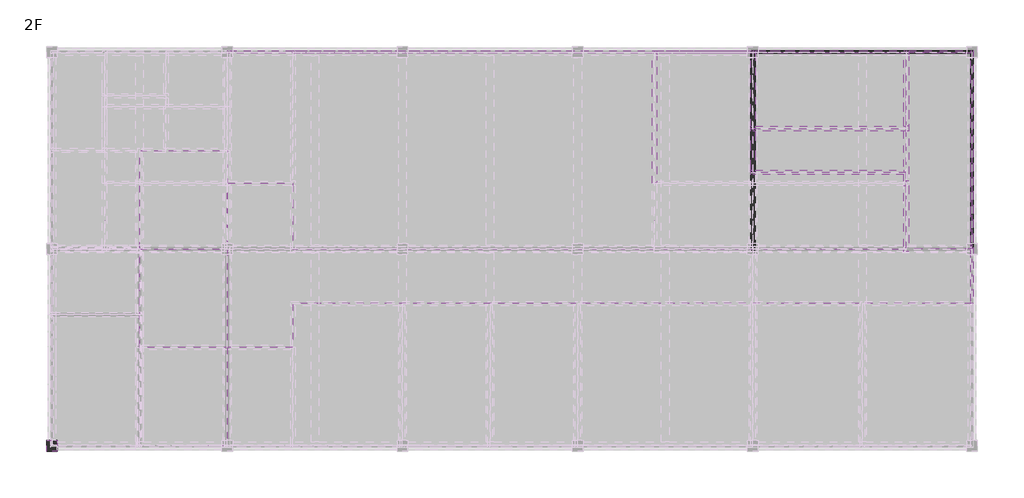
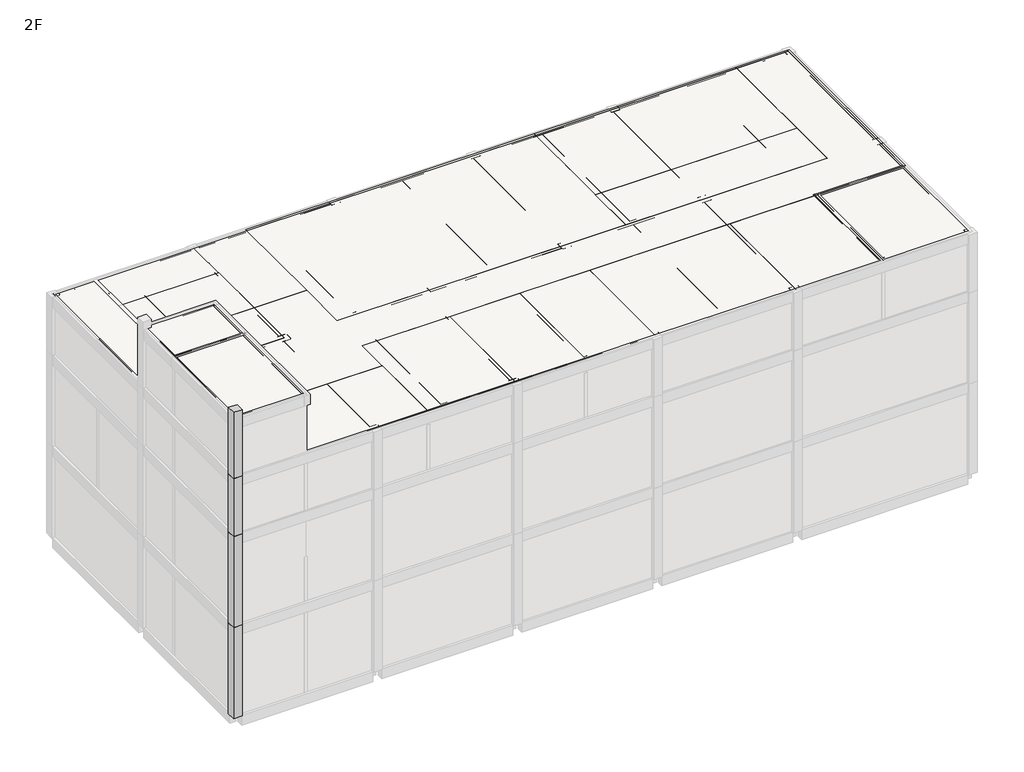
# One storey, part 3 of 7: 58 slabs, 19 walls, 4 columns.
# Revit data of these elements (continued)
# Element 71 (IfcWall, "WA211_Exterior-Cement Brick-90mm") (continued)
#   Base Offset = 0 mm
#   Unconnected Height = 3500 mm
#   wall height = 3500 mm
#   Phase Created = New Construction
#   Base Constraint = 4F
#   Materials on its faces: "Default Wall", "A04AS164-00001_Plastering_Ext", "A04AS164-00002_Plastering_Int"
# Element 73 (IfcWall, "WA221_Interior-Cement Block-190mm")
#   Top Offset = 0 mm
#   Base Offset = 0 mm
#   Unconnected Height = 5500 mm
#   wall height = 5500 mm
#   Phase Created = New Construction
#   Base Constraint = 2F
#   Materials on its faces: "A04AS164-00002_Plastering_Int", "Default Wall", "A04AS164-00001_Plastering_Ext"
# Element 74 (IfcWall, "WA221_Interior-Cement Block-190mm")
#   Top Offset = 0 mm
#   Base Offset = 0 mm
#   Unconnected Height = 3400 mm
#   wall height = 3400 mm
#   Phase Created = New Construction
#   Base Constraint = 3F
#   Materials on its faces: "Default Wall", "A04AS164-00002_Plastering_Int", "A04AS164-00001_Plastering_Ext"
# Element 75 (IfcWall, "WA221_Interior-Cement Block-190mm")
#   Top Offset = 0 mm
#   Base Offset = 0 mm
#   Unconnected Height = 3400 mm
#   wall height = 3400 mm
#   Phase Created = New Construction
#   Base Constraint = 3F
#   Materials on its faces: "Default Wall", "A04AS164-00002_Plastering_Int"
# Elements 76, 78 (IfcWall, "WA221_Interior-Cement Block-190mm")
#   Top Offset = 0 mm
#   Base Offset = 0 mm
#   Unconnected Height = 2700 mm
#   wall height = 2700 mm
#   Phase Created = New Construction
#   Base Constraint = 3F
#   Materials on its faces: "A04AS164-00002_Plastering_Int", "Default Wall"
# Element 77 (IfcWall, "WA221_Interior-Cement Block-190mm")
#   Top Offset = 0 mm
#   Base Offset = 0 mm
#   Unconnected Height = 2700 mm
#   wall height = 2700 mm
#   Phase Created = New Construction
#   Base Constraint = 3F
#   Materials on its faces: "Default Wall", "A04AS164-00002_Plastering_Int", "A04AS164-00001_Plastering_Ext"
# Elements 79, 80 (IfcWall, "WA221_Interior-Cement Block-190mm")
#   Top Offset = 0 mm
#   Base Offset = 0 mm
#   Unconnected Height = 2700 mm
#   wall height = 2700 mm
#   Phase Created = New Construction
#   Base Constraint = 4F
#   Materials on its faces: "Default Wall", "A04AS164-00002_Plastering_Int", "A04AS164-00001_Plastering_Ext"
# Element 81 (IfcWall, "WA221_Interior-Cement Block-190mm")
#   Top Offset = 0 mm
#   Base Offset = 0 mm
#   Unconnected Height = 2700 mm
#   wall height = 2700 mm
#   Phase Created = New Construction
#   Base Constraint = 4F
#   Materials on its faces: "A04AS164-00002_Plastering_Int", "Default Wall"
# Materials
#   "A03AE056-00001_Bitumen/Bituminous/Asphalt Coating": class "Generic", colour RGB 17 17 17, transparency 0, Description = "Damp-proofing", W00) Work Master Code = "A03AE056-00001", W01) Work Master_Lv1 = "Concrete Work", W02) Work Master_Lv2 = "Concrete Protective Coating (U/G)", W03) Work Master_Spec.1 = "Bitumen/Bituminous/Asphalt Coating", Cost = 0
#   "A03AC035-00001_Form Work (3 times in use)_Flat": class "Wood", colour RGB 149 120 74, transparency 0, Description = "Plywood", W00) Work Master Code = "A03AC035-00001", W01) Work Master_Lv1 = "Concrete Work", W02) Work Master_Lv2 = "Substructure Work", W03) Work Master_Spec.1 = "Form Work (3 times in use)", W04) Work Master_Spec.2 = "Flat Form", W05) Work Master_Spec.3 = "Dressed Lumber, Plywood or Steel Form(Wood Planks are not Allowed) incl. Chamfer", Cost = 0
#   "A03AC032-00007_Structural Concrete_Type1_25MPa-30Mpa": class "Concrete", colour RGB 176 176 176, transparency 0, Keynote = "09910.A1", Description = "Reinf. Conc.", W00) Work Master Code = "A03AC032-00007", W01) Work Master_Lv1 = "Concrete Work", W02) Work Master_Lv2 = "Substructure Work", W03) Work Master_Spec.1 = "Structural Concrete", W04) Work Master_Spec.2 = "Cement Type-1", W05) Work Master_Spec.3 = "25MPa < F'c (Cylinder Strength) ≤ 30MPa", Cost = 0
#   "14200-030101_Concrete Pouring": class "Concrete", colour RGB 176 176 176, transparency 0, Description = "Reinf. Conc.", W00) Work Master Code = "14200-030101", W01) Work Master_Lv1 = "Concrete Work", W02) Work Master_Lv2 = "Building/Shelter Foundation Work", W03) Work Master_Spec.1 = "Concrete Pouring", W04) Work Master_Spec.2 = "F'c (Cylinder Strength) > 35MPa", W05) Work Master_Spec.3 = "Cement Type-1", Cost = 0
#   "A04AL081-00001_Skirt_Acrylic Emulsion Paint": class "Finish", colour RGB 128 128 64, transparency 0, Description = "Plastic", W00) Work Master Code = "A04AL081-00001", W01) Work Master_Lv1 = "Finishing Work", W02) Work Master_Lv2 = "Painting Work", W03) Work Master_Spec.1 = "Skirt Painting", W04) Work Master_Spec.2 = "Acrylic Emulsion Paint", W05) Work Master_Spec.3 = "100mm≤H<150mm", Cost = 0
#   "A04AL077-00001_Ext Wall Painting_Acrylic Emulsion Paint": class "Finish", colour RGB 128 128 64, transparency 0, Description = "Plastic", W00) Work Master Code = "A04AL077-00001", W01) Work Master_Lv1 = "Finishing Work", W02) Work Master_Lv2 = "Painting Work", W03) Work Master_Spec.1 = "External Wall Painting", W04) Work Master_Spec.2 = "Acrylic Emulsion Paint", Cost = 0
#   "A04AS164-00001_Plastering_Ext": class "Concrete", colour RGB 183 186 184, transparency 0, W00) Work Master Code = "A04AS164-00001", W01) Work Master_Lv1 = "Finishing Work", W02) Work Master_Lv2 = "Plastering Work", W03) Work Master_Spec.1 = "Plastering", W04) Work Master_Spec.2 = "for External Masonry Wall", Cost = 0
#   "A04AK073-00001_Concrete Brick_0.5B": class "Concrete", colour RGB 180 180 180, transparency 0, Description = "Conc. Block", W00) Work Master Code = "A04AK073-00001", W01) Work Master_Lv1 = "Finishing Work", W02) Work Master_Lv2 = "Masonry Work", W03) Work Master_Spec.1 = "Concrete Brick", W04) Work Master_Spec.2 = "[0.5B] w/ All Reinf.(Lath, Steel Tie, Anchor Bar, Mortar, ETC.), Filler, Sealant, Lintel/Sill for Opening, ETC.", Cost = 0
#   "A04AS164-00002_Plastering_Int": class "Concrete", colour RGB 183 186 184, transparency 0, Description = "LATEX PAINT ON THK.15 CEMENT PLASTER", W00) Work Master Code = "A04AS164-00002", W01) Work Master_Lv1 = "Finishing Work", W02) Work Master_Lv2 = "Plastering Work", W03) Work Master_Spec.1 = "Plastering", W04) Work Master_Spec.2 = "for Internal Masonry Wall", Cost = 0
#   "A04AL078-00002_Int Wall Painting_Water Emulsion Paint": class "Finish", colour RGB 128 128 64, transparency 0, Description = "Plastic", W00) Work Master Code = "A04AL078-00002", W01) Work Master_Lv1 = "Finishing Work", W02) Work Master_Lv2 = "Painting Work", W03) Work Master_Spec.1 = "Internal Wall Painting", W04) Work Master_Spec.2 = "Water Emulsion Paint", Cost = 0
#   "A04AK069-00002_Reinforced Concrete Block_THK 100-200mm": class "Concrete", colour RGB 180 180 180, transparency 0, Description = "Conc. Block", W00) Work Master Code = "A04AK069-00002", W01) Work Master_Lv1 = "Finishing Work", W02) Work Master_Lv2 = "Masonry Work", W03) Work Master_Spec.1 = "Reinforced Concrete Block", W04) Work Master_Spec.2 = "w/ All Reinf.(Lath, Steel Tie, Anchor Bar, Mortar, ETC.), Filler, Sealant, Lintel/Sill for Opening, ETC.", W05) Work Master_Spec.3 = "100mm<THK≤200mm", Cost = 0
#   "콘크리트 - 현장타설 콘크리트": class "콘크리트", colour RGB 192 192 192, transparency 0
#   "Default Wall": class "Miscellaneous", colour RGB 80 80 80, transparency 0
